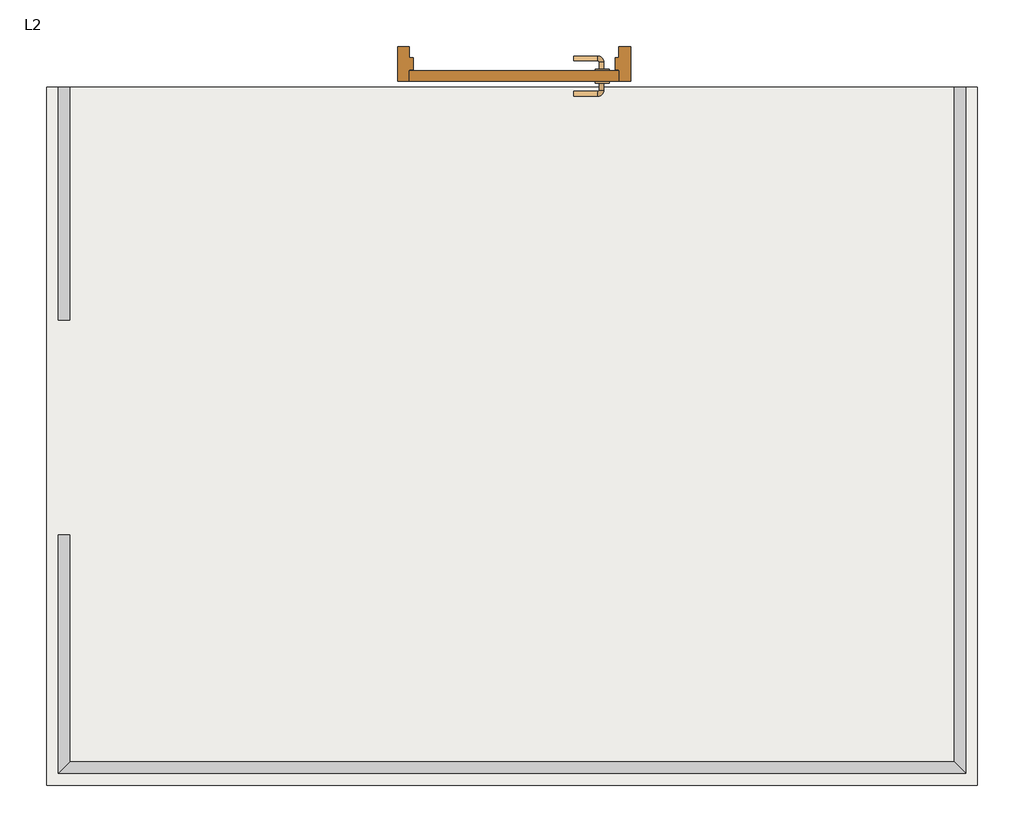
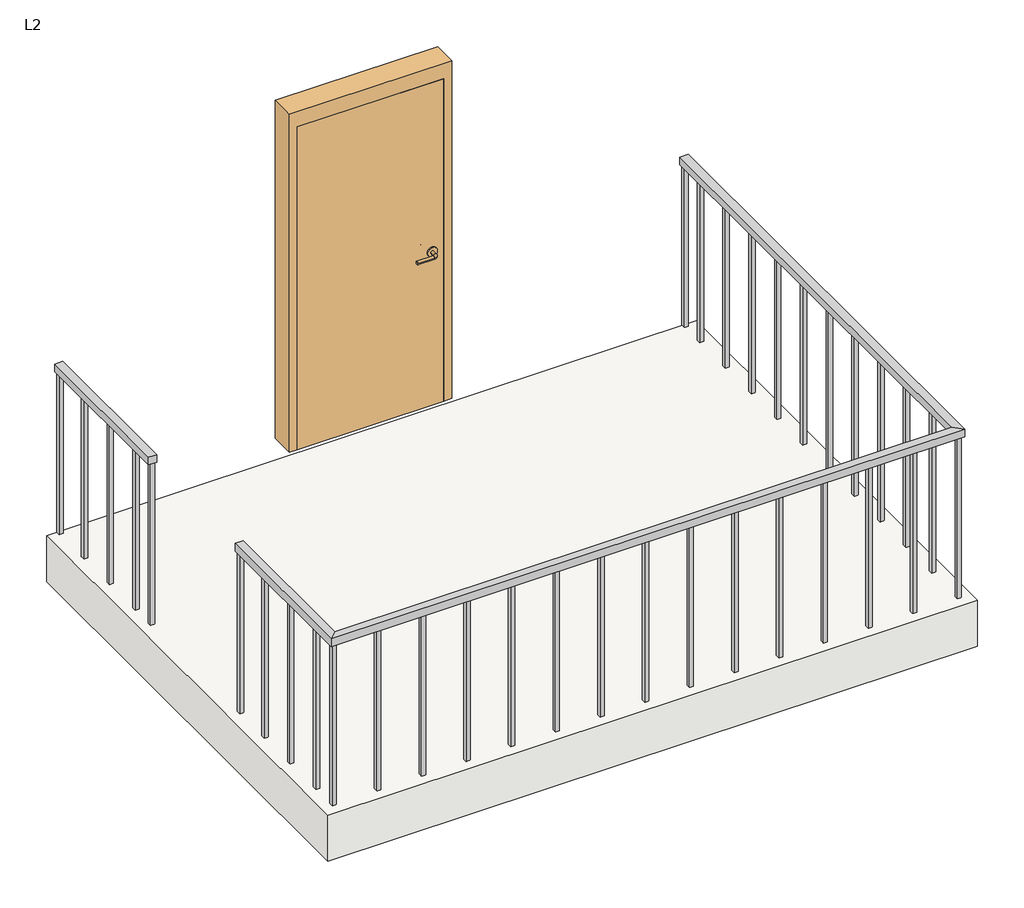
# One storey: 2 railings, 1 door, 1 slab.
"""IFC4 building model written with IfcOpenShell, lengths in millimetres."""

import ifcopenshell
import ifcopenshell.guid

model = None  # the IFC model being written
_history = None  # IfcOwnerHistory: only IFC2X3 demands one
_inside = {}  # id of a spatial element -> (the spatial element, [elements in it])
_under = {}  # id of a project, library or spatial element -> (it, [spatial elements below it])
_declared = {}  # id of a project -> (the project, [libraries it declares])
_typed = {}  # id of a type object -> (the type object, [elements of that type])
_made_of = {}  # id of a material, layer set ... -> (it, [elements and type objects made of it])


def new_model(schema):
    """Start an empty IFC model of exactly this schema.

    Asked for "IFC4X3", IfcOpenShell would pick the latest addendum, in which some entities
    have other attributes; the version numbers below select the first issue.
    IFC2X3 requires an IfcOwnerHistory on every rooted entity: one is made here for all.
    """
    global model, _history
    if schema == "IFC4X3":
        model = ifcopenshell.file(schema_version=(4, 3, 0, 0))
    else:
        model = ifcopenshell.file(schema=schema)
    _inside.clear()
    _under.clear()
    _declared.clear()
    _typed.clear()
    _made_of.clear()
    _history = None
    if model.schema == "IFC2X3":
        org = make("IfcOrganization", Name="unknown")
        user = make(
            "IfcPersonAndOrganization",
            ThePerson=make("IfcPerson", FamilyName="unknown"),
            TheOrganization=org,
        )
        app = make(
            "IfcApplication",
            ApplicationDeveloper=org,
            Version="unknown",
            ApplicationFullName="unknown",
            ApplicationIdentifier="unknown",
        )
        _history = make(
            "IfcOwnerHistory",
            OwningUser=user,
            OwningApplication=app,
            ChangeAction="ADDED",
            CreationDate=0,
        )
    return model


def make(cls, **values):
    """One entity of the class cls with the attributes given. An attribute that is None is left unset."""
    return model.create_entity(
        cls, **{name: value for name, value in values.items() if value is not None}
    )


def rooted(cls, **values):
    """An entity with a GlobalId (a new one), such as an element, a storey or a relation."""
    return make(cls, GlobalId=ifcopenshell.guid.new(), OwnerHistory=_history, **values)


def si_unit(unit_type, name, prefix=None):
    """IfcSIUnit, for example si_unit("LENGTHUNIT", "METRE", prefix="MILLI")."""
    return make("IfcSIUnit", UnitType=unit_type, Prefix=prefix, Name=name)


def assignment(units):
    """IfcUnitAssignment: the units of a project."""
    return None if units is None else make("IfcUnitAssignment", Units=units)


def point(xyz):
    """IfcCartesianPoint."""
    return None if xyz is None else make("IfcCartesianPoint", Coordinates=xyz)


def direction(xyz):
    """IfcDirection."""
    return None if xyz is None else make("IfcDirection", DirectionRatios=xyz)


def frame(location, z_axis=None, x_axis=None):
    """IfcAxis2Placement3D, a coordinate frame: its origin and axes. An axis left out is left unset."""
    return make(
        "IfcAxis2Placement3D",
        Location=point(location),
        Axis=direction(z_axis),
        RefDirection=direction(x_axis),
    )


def frame_2d(location, x_axis=None):
    """IfcAxis2Placement2D, a coordinate frame in the plane: its origin and x axis."""
    return make(
        "IfcAxis2Placement2D", Location=point(location), RefDirection=direction(x_axis)
    )


def origin():
    """The frame at (0, 0, 0) with its axes left unset."""
    return frame((0.0, 0.0, 0.0))


def origin_with_axes():
    """The frame at (0, 0, 0) with the z axis (0, 0, 1) and the x axis (1, 0, 0) written out."""
    return frame((0.0, 0.0, 0.0), z_axis=(0.0, 0.0, 1.0), x_axis=(1.0, 0.0, 0.0))


def place(relative_to, where):
    """IfcLocalPlacement: puts the frame where relative to a parent placement (None: the world)."""
    return make(
        "IfcLocalPlacement", PlacementRelTo=relative_to, RelativePlacement=where
    )


def context(
    kind, dimensions, precision=None, world=None, true_north=None, identifier=None
):
    """IfcGeometricRepresentationContext, for example the 3D "Model" context."""
    return make(
        "IfcGeometricRepresentationContext",
        ContextIdentifier=identifier,
        ContextType=kind,
        CoordinateSpaceDimension=dimensions,
        Precision=precision,
        WorldCoordinateSystem=world,
        TrueNorth=true_north,
    )


def project(units=None, contexts=None):
    """IfcProject with its units and contexts."""
    return rooted(
        "IfcProject",
        Name="project",
        RepresentationContexts=contexts,
        UnitsInContext=assignment(units),
    )


def spatial(cls, under=None, at=None, **own):
    """A site, building, storey or space (cls), placed at a placement, below another one or the project."""
    s = rooted(cls, ObjectPlacement=at, **own)
    if under is not None:
        _under.setdefault(under.id(), (under, []))[1].append(s)
    return s


def polyline(points):
    """IfcPolyline through the points."""
    return make("IfcPolyline", Points=[point(p) for p in points])


def circle_curve(where, radius):
    """IfcCircle in the frame where."""
    return make("IfcCircle", Position=where, Radius=radius)


def ellipse_curve(where, semi_axis1, semi_axis2):
    """IfcEllipse in the frame where."""
    return make(
        "IfcEllipse", Position=where, SemiAxis1=semi_axis1, SemiAxis2=semi_axis2
    )


def trimmed(basis, trim1, trim2, sense, master):
    """IfcTrimmedCurve: the piece of a basis curve between two trims."""
    return make(
        "IfcTrimmedCurve",
        BasisCurve=basis,
        Trim1=trim1,
        Trim2=trim2,
        SenseAgreement=sense,
        MasterRepresentation=master,
    )


def segment(curve, same_sense, transition):
    """IfcCompositeCurveSegment."""
    return make(
        "IfcCompositeCurveSegment",
        Transition=transition,
        SameSense=same_sense,
        ParentCurve=curve,
    )


def composite_curve(segments, self_intersect=None):
    """IfcCompositeCurve: segments joined end to end."""
    return make("IfcCompositeCurve", Segments=segments, SelfIntersect=self_intersect)


def outline(outer, holes=None, kind="AREA"):
    """IfcArbitraryClosedProfileDef: a profile drawn as a closed curve; with holes, ...WithVoids."""
    if holes is None:
        return make("IfcArbitraryClosedProfileDef", ProfileType=kind, OuterCurve=outer)
    return make(
        "IfcArbitraryProfileDefWithVoids",
        ProfileType=kind,
        OuterCurve=outer,
        InnerCurves=holes,
    )


def extrude(swept, where, along, depth):
    """IfcExtrudedAreaSolid: the profile swept, set in the frame where, extruded along a direction by depth."""
    return make(
        "IfcExtrudedAreaSolid",
        SweptArea=swept,
        Position=where,
        ExtrudedDirection=direction(along),
        Depth=depth,
    )


def faces_of(points, faces, orient=None, outer=None):
    """IfcFace entities. A face is a list of loops; a loop is a list of indices into points, from 0.

    orient and outer hold one flag for each loop. By default every Orientation is true, the
    first loop of a face is its IfcFaceOuterBound and the others are IfcFaceBound.
    """
    made = []
    for i, loops in enumerate(faces):
        bounds = []
        for j, loop in enumerate(loops):
            is_outer = j == 0 if outer is None else outer[i][j]
            bounds.append(
                make(
                    "IfcFaceOuterBound" if is_outer else "IfcFaceBound",
                    Bound=make("IfcPolyLoop", Polygon=[points[k] for k in loop]),
                    Orientation=True if orient is None else orient[i][j],
                )
            )
        made.append(make("IfcFace", Bounds=bounds))
    return made


def faceted_brep(points, faces, orient=None, outer=None, voids=None):
    """IfcFacetedBrep: a solid bounded by flat faces; with voids (closed shells), ...WithVoids."""
    shared = [point(p) for p in points]
    hull = make("IfcClosedShell", CfsFaces=faces_of(shared, faces, orient, outer))
    if voids is None:
        return make("IfcFacetedBrep", Outer=hull)
    return make(
        "IfcFacetedBrepWithVoids",
        Outer=hull,
        Voids=[
            make(cls, CfsFaces=faces_of(shared, fs, o, b)) for cls, fs, o, b in voids
        ],
    )


def shape(context_of_items, identifier, shape_type, items):
    """IfcShapeRepresentation: the items that make up one representation, for example the "Body"."""
    return make(
        "IfcShapeRepresentation",
        ContextOfItems=context_of_items,
        RepresentationIdentifier=identifier,
        RepresentationType=shape_type,
        Items=items,
    )


def source(mapping_origin, context_of_items, identifier, shape_type, items):
    """IfcRepresentationMap: a shape defined once, which mapped items show again and again."""
    return make(
        "IfcRepresentationMap",
        MappingOrigin=mapping_origin,
        MappedRepresentation=shape(context_of_items, identifier, shape_type, items),
    )


def transform(
    local_origin,
    x_axis=None,
    y_axis=None,
    z_axis=None,
    scale=None,
    scale2=None,
    scale3=None,
    uniform=True,
):
    """IfcCartesianTransformationOperator3D, or its non-uniform kind. x_axis, y_axis, z_axis: its Axis1, 2, 3."""
    if uniform:
        return make(
            "IfcCartesianTransformationOperator3D",
            Axis1=direction(x_axis),
            Axis2=direction(y_axis),
            LocalOrigin=point(local_origin),
            Scale=scale,
            Axis3=direction(z_axis),
        )
    return make(
        "IfcCartesianTransformationOperator3DnonUniform",
        Axis1=direction(x_axis),
        Axis2=direction(y_axis),
        LocalOrigin=point(local_origin),
        Scale=scale,
        Axis3=direction(z_axis),
        Scale2=scale2,
        Scale3=scale3,
    )


def mapped(mapping_source, mapping_target):
    """IfcMappedItem: shows the shape of a source again, moved by a transform."""
    return make(
        "IfcMappedItem", MappingSource=mapping_source, MappingTarget=mapping_target
    )


def made_of(thing, what):
    """Note that an element or type object is made of a material, layer set ...; save() writes the relation."""
    if what is not None:
        _made_of.setdefault(what.id(), (what, []))[1].append(thing)
    return thing


def element(
    cls,
    number,
    at=None,
    inside=None,
    cuts=None,
    type_object=None,
    material=None,
    context=None,
    identifier="Body",
    shape_type=None,
    held_by="IfcProductDefinitionShape",
    body=None,
    shapes=None,
    **own,
):
    """One element of the class cls, such as IfcWall. Its Tag is "e" and its number.

    at: its placement. inside: the storey or other place that contains it. cuts: it is an
    opening in that element (IfcRelVoidsElement). A single representation is given by context,
    identifier, shape_type and body (its items); several are given by shapes. held_by: the class
    of the entity that holds the representations. save() writes the other relations.
    """
    e = rooted(cls, Tag="e%d" % number, ObjectPlacement=at, **own)
    if body is not None:
        shapes = [shape(context, identifier, shape_type, body)]
    if shapes is not None:
        e.Representation = make(held_by, Representations=shapes)
    if inside is not None:
        _inside.setdefault(inside.id(), (inside, []))[1].append(e)
    if cuts is not None:
        rooted(
            "IfcRelVoidsElement", RelatingBuildingElement=cuts, RelatedOpeningElement=e
        )
    if type_object is not None:
        _typed.setdefault(type_object.id(), (type_object, []))[1].append(e)
    return made_of(e, material)


def aggregate(whole, parts):
    """IfcRelAggregates: a whole, such as a stair, and the parts it consists of."""
    return rooted("IfcRelAggregates", RelatingObject=whole, RelatedObjects=parts)


def save(model, path):
    """Write the relations noted so far, then the file.

    IfcRelAggregates (storeys below a building ...), IfcRelContainedInSpatialStructure (elements
    in a storey), IfcRelDefinesByType, IfcRelAssociatesMaterial and IfcRelDeclares: one each for
    every whole, place, type object, material and project.
    """
    for whole, parts in _under.values():
        aggregate(whole, parts)
    for where, things in _inside.values():
        rooted(
            "IfcRelContainedInSpatialStructure",
            RelatedElements=things,
            RelatingStructure=where,
        )
    for kind, things in _typed.values():
        rooted("IfcRelDefinesByType", RelatedObjects=things, RelatingType=kind)
    for what, things in _made_of.values():
        rooted("IfcRelAssociatesMaterial", RelatedObjects=things, RelatingMaterial=what)
    for by, libraries in _declared.values():
        rooted("IfcRelDeclares", RelatingContext=by, RelatedDefinitions=libraries)
    model.write(path)


def plane_surface(at):
    """IfcPlane: the flat surface through the origin of the frame at, square to its z axis."""
    return make("IfcPlane", Position=at)


def cylinder_surface(at, radius):
    """IfcCylindricalSurface: all points at the distance radius from the z axis of the frame at."""
    return make("IfcCylindricalSurface", Position=at, Radius=radius)


def revolved_surface(curve, axis_point, axis_direction):
    """IfcSurfaceOfRevolution: the curve turned about the line through axis_point along axis_direction."""
    return make(
        "IfcSurfaceOfRevolution",
        SweptCurve=make("IfcArbitraryOpenProfileDef", ProfileType="CURVE", Curve=curve),
        AxisPosition=make("IfcAxis1Placement", Location=point(axis_point), Axis=direction(axis_direction)),
    )


def advanced_brep(points, edges, surfaces, faces):
    """IfcAdvancedBrep: a solid bounded by faces that lie on surfaces and meet in shared edges.

    An edge is (start, end): straight between two places in points (the first is 0);
    or (start, end, curve); or (start, end, curve, False) where it runs against its curve.
    A face is (place in surfaces, loops), or (place, loops, False) where it looks against
    its surface's normal. A loop lists edges by number (the first is 1), with a minus sign
    where the edge is run from its end to its start. The first loop is the outer one.
    """
    corners = [point(p) for p in points]
    vertices = [make("IfcVertexPoint", VertexGeometry=c) for c in corners]
    made = []
    for start, end, *more in edges:
        made.append(
            make(
                "IfcEdgeCurve",
                EdgeStart=vertices[start],
                EdgeEnd=vertices[end],
                EdgeGeometry=more[0] if more else make("IfcPolyline", Points=[corners[start], corners[end]]),
                SameSense=more[1] if len(more) > 1 else True,
            )
        )
    hull = []
    for where, loops, *sense in faces:
        bounds = []
        for j, loop in enumerate(loops):
            ring = [make("IfcOrientedEdge", EdgeElement=made[abs(k) - 1], Orientation=k > 0) for k in loop]
            bounds.append(
                make(
                    "IfcFaceOuterBound" if j == 0 else "IfcFaceBound",
                    Bound=make("IfcEdgeLoop", EdgeList=ring),
                    Orientation=True,
                )
            )
        hull.append(make("IfcAdvancedFace", Bounds=bounds, FaceSurface=surfaces[where], SameSense=sense[0] if sense else True))
    return make("IfcAdvancedBrep", Outer=make("IfcClosedShell", CfsFaces=hull))


def m_door_passage_single_flush_900_x_2100mm_f70d95c9(model_context):
    return source(origin(), model_context, "Body", "SolidModel", [
        advanced_brep(
        [(-384.990625, 3.35, 1000.0), (-364.990625, 3.35, 1000.0), (-364.990625, -26.65, 1000.0), (-384.990625, -26.65, 1000.0), (-359.990625, -31.65, 1000.0), (-359.990625, -51.65, 1000.0), (-254.990625, -51.65, 1000.0), (-254.990625, -31.65, 1000.0)],
        [
            (0, 1, circle_curve(frame((-374.990625, 3.35, 1000.0), z_axis=(0.0, 1.0, 0.0), x_axis=(1.0, 0.0, 0.0)), 10.0)),
            (1, 0, circle_curve(frame((-374.990625, 3.35, 1000.0), z_axis=(0.0, 1.0, 0.0), x_axis=(1.0, 0.0, 0.0)), 10.0)),
            (1, 2),
            (2, 3, circle_curve(frame((-374.990625, -26.65, 1000.0), z_axis=(0.0, 1.0, 0.0), x_axis=(1.0, 0.0, 0.0)), 10.0)),
            (3, 0),
            (3, 2, circle_curve(frame((-374.990625, -26.65, 1000.0), z_axis=(0.0, 1.0, 0.0), x_axis=(1.0, 0.0, 0.0)), 10.0)),
            (4, 5, circle_curve(frame((-359.990625, -41.65, 1000.0), z_axis=(-1.0, 0.0, 0.0), x_axis=(0.0, 1.0, 0.0)), 10.0)),
            (5, 3, circle_curve(frame((-359.990625, -26.65, 1000.0), z_axis=(0.0, 0.0, -1.0), x_axis=(-1.0, 0.0, 0.0)), 25.0)),
            (2, 4, circle_curve(frame((-359.990625, -26.65, 1000.0), z_axis=(0.0, 0.0, 1.0), x_axis=(-1.0, 0.0, 0.0)), 5.0)),
            (5, 4, circle_curve(frame((-359.990625, -41.65, 1000.0), z_axis=(-1.0, 0.0, 0.0), x_axis=(0.0, 1.0, 0.0)), 10.0)),
            (6, 7, circle_curve(frame((-254.990625, -41.65, 1000.0), z_axis=(1.0, 0.0, 0.0), x_axis=(0.0, 1.0, 0.0)), 10.0)),
            (7, 6, circle_curve(frame((-254.990625, -41.65, 1000.0), z_axis=(1.0, 0.0, 0.0), x_axis=(0.0, 1.0, 0.0)), 10.0)),
            (4, 7),
            (6, 5),
        ],
        [
            plane_surface(frame((-374.990625, 3.35, 1000.0), z_axis=(0.0, 1.0, 0.0), x_axis=(0.0, 0.0, 1.0))),
            cylinder_surface(frame((-374.990625, 3.35, 1000.0), z_axis=(0.0, 1.0, 0.0), x_axis=(1.0, 0.0, 0.0)), 10.0),
            revolved_surface(trimmed(ellipse_curve(frame((-374.990625, -26.65, 1000.0), z_axis=(0.0, -1.0, 0.0), x_axis=(1.0, 0.0, 0.0)), 10.0, 10.0), [point((-384.990625, -26.65, 1000.0))], [point((-364.990625, -26.65, 1000.0))], True, "CARTESIAN"), (-359.990625, -26.65, 1000.0), (0.0, 0.0, -1.0)),
            revolved_surface(trimmed(ellipse_curve(frame((-374.990625, -26.65, 1000.0), z_axis=(0.0, -1.0, 0.0), x_axis=(1.0, 0.0, 0.0)), 10.0, 10.0), [point((-364.990625, -26.65, 1000.0))], [point((-384.990625, -26.65, 1000.0))], True, "CARTESIAN"), (-359.990625, -26.65, 1000.0), (0.0, 0.0, -1.0)),
            plane_surface(frame((-254.990625, -41.65, 1000.0), z_axis=(1.0, 0.0, 0.0), x_axis=(0.0, 0.0, 1.0))),
            cylinder_surface(frame((-359.990625, -41.65, 1000.0), z_axis=(-1.0, 0.0, 0.0), x_axis=(0.0, 1.0, 0.0)), 10.0),
        ],
        [
            (0, [[1, 2]]),
            (1, [[3, 4, 5, -2]]),
            (1, [[-5, 6, -3, -1]]),
            (2, [[7, 8, -4, 9]]),
            (3, [[10, -9, -6, -8]]),
            (4, [[11, 12]]),
            (5, [[13, -11, 14, -7]]),
            (5, [[-14, -12, -13, -10]]),
        ],
    ),
        extrude(outline(composite_curve([segment(trimmed(circle_curve(frame_2d((1000.0, -377.490625)), 30.0), [point((1000.0, -407.490625))], [point((1000.0, -347.490625))], False, "CARTESIAN"), True, "CONTINUOUS"), segment(trimmed(circle_curve(frame_2d((1000.0, -377.490625)), 30.0), [point((1000.0, -347.490625))], [point((1000.0, -407.490625))], False, "CARTESIAN"), True, "CONTINUOUS")], self_intersect=False)), frame((0.0, 3.35, 0.0), z_axis=(0.0, 1.0, 0.0), x_axis=(0.0, 0.0, 1.0)), (0.0, 0.0, 1.0), 8.0),
        advanced_brep(
        [(-384.990625, 64.35, 1000.0), (-364.990625, 64.35, 1000.0), (-384.990625, 94.35, 1000.0), (-364.990625, 94.35, 1000.0), (-359.990625, 99.35, 1000.0), (-359.990625, 119.35, 1000.0), (-254.990625, 119.35, 1000.0), (-254.990625, 99.35, 1000.0)],
        [
            (0, 1, circle_curve(frame((-374.990625, 64.35, 1000.0), z_axis=(0.0, -1.0, 0.0), x_axis=(1.0, 0.0, 0.0)), 10.0)),
            (1, 0, circle_curve(frame((-374.990625, 64.35, 1000.0), z_axis=(0.0, -1.0, 0.0), x_axis=(1.0, 0.0, 0.0)), 10.0)),
            (0, 2),
            (2, 3, circle_curve(frame((-374.990625, 94.35, 1000.0), z_axis=(0.0, -1.0, 0.0), x_axis=(1.0, 0.0, 0.0)), 10.0)),
            (3, 1),
            (3, 2, circle_curve(frame((-374.990625, 94.35, 1000.0), z_axis=(0.0, -1.0, 0.0), x_axis=(1.0, 0.0, 0.0)), 10.0)),
            (4, 3, circle_curve(frame((-359.990625, 94.35, 1000.0), z_axis=(0.0, 0.0, 1.0), x_axis=(-1.0, 0.0, 0.0)), 5.0)),
            (2, 5, circle_curve(frame((-359.990625, 94.35, 1000.0), z_axis=(0.0, 0.0, -1.0), x_axis=(-1.0, 0.0, 0.0)), 25.0)),
            (5, 4, circle_curve(frame((-359.990625, 109.35, 1000.0), z_axis=(-1.0, 0.0, 0.0), x_axis=(0.0, -1.0, 0.0)), 10.0)),
            (4, 5, circle_curve(frame((-359.990625, 109.35, 1000.0), z_axis=(-1.0, 0.0, 0.0), x_axis=(0.0, -1.0, 0.0)), 10.0)),
            (6, 7, circle_curve(frame((-254.990625, 109.35, 1000.0), z_axis=(1.0, 0.0, 0.0), x_axis=(0.0, -1.0, 0.0)), 10.0)),
            (7, 6, circle_curve(frame((-254.990625, 109.35, 1000.0), z_axis=(1.0, 0.0, 0.0), x_axis=(0.0, -1.0, 0.0)), 10.0)),
            (5, 6),
            (7, 4),
        ],
        [
            plane_surface(frame((-374.990625, 64.35, 1000.0), z_axis=(0.0, -1.0, 0.0), x_axis=(0.0, 0.0, 1.0))),
            cylinder_surface(frame((-374.990625, 64.35, 1000.0), z_axis=(0.0, -1.0, 0.0), x_axis=(1.0, 0.0, 0.0)), 10.0),
            revolved_surface(trimmed(ellipse_curve(frame((-374.990625, 94.35, 1000.0), z_axis=(0.0, -1.0, 0.0), x_axis=(1.0, 0.0, 0.0)), 10.0, 10.0), [point((-384.990625, 94.35, 1000.0))], [point((-364.990625, 94.35, 1000.0))], True, "CARTESIAN"), (-359.990625, 94.35, 1000.0), (0.0, 0.0, -1.0)),
            revolved_surface(trimmed(ellipse_curve(frame((-374.990625, 94.35, 1000.0), z_axis=(0.0, -1.0, 0.0), x_axis=(1.0, 0.0, 0.0)), 10.0, 10.0), [point((-364.990625, 94.35, 1000.0))], [point((-384.990625, 94.35, 1000.0))], True, "CARTESIAN"), (-359.990625, 94.35, 1000.0), (0.0, 0.0, -1.0)),
            plane_surface(frame((-254.990625, 109.35, 1000.0), z_axis=(1.0, 0.0, 0.0), x_axis=(0.0, 0.0, 1.0))),
            cylinder_surface(frame((-359.990625, 109.35, 1000.0), z_axis=(-1.0, 0.0, 0.0), x_axis=(0.0, -1.0, 0.0)), 10.0),
        ],
        [
            (0, [[1, 2]]),
            (1, [[-1, 3, 4, 5]]),
            (1, [[-2, -5, 6, -3]]),
            (2, [[7, -4, 8, 9]]),
            (3, [[-8, -6, -7, 10]]),
            (4, [[11, 12]]),
            (5, [[-9, 13, -12, 14]]),
            (5, [[-10, -14, -11, -13]]),
        ],
    ),
        extrude(outline(composite_curve([segment(trimmed(circle_curve(frame_2d((1000.0, -377.490625)), 30.0), [point((1000.0, -407.490625))], [point((1000.0, -347.490625))], False, "CARTESIAN"), True, "CONTINUOUS"), segment(trimmed(circle_curve(frame_2d((1000.0, -377.490625)), 30.0), [point((1000.0, -347.490625))], [point((1000.0, -407.490625))], False, "CARTESIAN"), True, "CONTINUOUS")], self_intersect=False)), frame((0.0, 56.35, 0.0), z_axis=(0.0, 1.0, 0.0), x_axis=(0.0, 0.0, 1.0)), (0.0, 0.0, 1.0), 8.0),
        extrude(outline(polyline([(450.0, 11.35), (-450.0, 11.35), (-450.0, 56.35), (450.0, 56.35), (450.0, 11.35)])), origin_with_axes(), (0.0, 0.0, 1.0), 2100.0),
        faceted_brep([(450.0, 6.5875, 0.0), (450.0, 56.35, 0.0), (500.0, 56.35, 0.0), (500.0, -93.65, 0.0), (450.0, -93.65, 0.0), (450.0, -44.4375, 0.0), (434.125, -44.4375, 0.0), (434.125, 6.5875, 0.0), (450.0, 6.5875, 2100.0), (450.0, 56.35, 2100.0), (-450.0, 56.35, 2100.0), (-450.0, 56.35, 0.0), (-500.0, 56.35, 0.0), (-500.0, 56.35, 2200.0), (500.0, 56.35, 2200.0), (500.0, -93.65, 2200.0), (-500.0, -93.65, 2200.0), (-500.0, -93.65, 0.0), (-450.0, -93.65, 0.0), (-450.0, -93.65, 2100.0), (450.0, -93.65, 2100.0), (450.0, -44.4375, 2100.0), (-450.0, -44.4375, 2100.0), (-450.0, -44.4375, 0.0), (-434.125, -44.4375, 0.0), (-434.125, -44.4375, 2084.125), (434.125, -44.4375, 2084.125), (434.125, 6.5875, 2084.125), (-434.125, 6.5875, 2084.125), (-434.125, 6.5875, 0.0), (-450.0, 6.5875, 0.0), (-450.0, 6.5875, 2100.0)], [[[0, 1, 2, 3, 4, 5, 6, 7]], [[1, 0, 8, 9]], [[2, 1, 9, 10, 11, 12, 13, 14]], [[3, 2, 14, 15]], [[4, 3, 15, 16, 17, 18, 19, 20]], [[5, 4, 20, 21]], [[6, 5, 21, 22, 23, 24, 25, 26]], [[7, 6, 26, 27]], [[0, 7, 27, 28, 29, 30, 31, 8]], [[9, 8, 31, 10]], [[20, 19, 22, 21]], [[26, 25, 28, 27]], [[12, 11, 30, 29, 24, 23, 18, 17]], [[11, 10, 31, 30]], [[13, 12, 17, 16]], [[19, 18, 23, 22]], [[25, 24, 29, 28]], [[15, 14, 13, 16]]]),
    ])


model = new_model("IFC4")

# Units and contexts
model_context = context("Model", 3, world=origin())
ifc_project = project(units=[si_unit("LENGTHUNIT", "METRE", prefix="MILLI")], contexts=[model_context])

# Site, building, storey
site = spatial("IfcSite", under=ifc_project)
building = spatial("IfcBuilding", under=site)
storey = spatial("IfcBuildingStorey", under=building, Name="L2", Elevation=1200.0)

# Door
placement = place(None, origin())
m_door_passage_single_flush_900_x_2100mm_shape = m_door_passage_single_flush_900_x_2100mm_f70d95c9(model_context)
element("IfcDoor", 1, ObjectType="M_Door-Passage-Single-Flush : 900 x 2100mm", at=placement, inside=storey, context=model_context, shape_type="MappedRepresentation", body=[
    mapped(m_door_passage_single_flush_900_x_2100mm_shape, transform((752.7568, 2222.9207088, 1200.0), x_axis=(-1.0, 0.0, 0.0), y_axis=(0.0, -1.0, 0.0), z_axis=(0.0, 0.0, 1.0))),
])

# Railings
element("IfcRailing", 2, ObjectType="1100mm", at=placement, inside=storey, context=model_context, shape_type="SolidModel", body=[
    faceted_brep([(-1156.7682, 216.5707088, 2300.0), (-1156.7682, 216.5707088, 2250.0), (-1206.7682, 216.5707088, 2250.0), (-1206.7682, 216.5707088, 2300.0), (-1156.7682, -758.4292912, 2300.0), (-1156.7682, -758.4292912, 2250.0), (-1206.7682, -808.4292912, 2250.0), (-1206.7682, -808.4292912, 2300.0), (2643.2318, -758.4292912, 2300.0), (2643.2318, -758.4292912, 2250.0), (2693.2318, -808.4292912, 2250.0), (2693.2318, -808.4292912, 2300.0), (2643.2318, 2141.5707088, 2300.0), (2693.2318, 2141.5707088, 2300.0), (2693.2318, 2141.5707088, 2250.0), (2643.2318, 2141.5707088, 2250.0)], [[[0, 1, 2, 3]], [[1, 0, 4, 5]], [[2, 1, 5, 6]], [[3, 2, 6, 7]], [[0, 3, 7, 4]], [[5, 4, 8, 9]], [[6, 5, 9, 10]], [[7, 6, 10, 11]], [[4, 7, 11, 8]], [[12, 13, 14, 15]], [[9, 8, 12, 15]], [[10, 9, 15, 14]], [[11, 10, 14, 13]], [[8, 11, 13, 12]]]),
    extrude(outline(polyline([(2680.7318, 1954.0707088), (2655.7318, 1954.0707088), (2655.7318, 1979.0707088), (2680.7318, 1979.0707088), (2680.7318, 1954.0707088)])), frame((0.0, 0.0, 1200.0), z_axis=(0.0, 0.0, 1.0), x_axis=(1.0, 0.0, 0.0)), (0.0, 0.0, 1.0), 1050.0),
    extrude(outline(polyline([(2680.7318, 1679.0707088), (2655.7318, 1679.0707088), (2655.7318, 1704.0707088), (2680.7318, 1704.0707088), (2680.7318, 1679.0707088)])), frame((0.0, 0.0, 1200.0), z_axis=(0.0, 0.0, 1.0), x_axis=(1.0, 0.0, 0.0)), (0.0, 0.0, 1.0), 1050.0),
    extrude(outline(polyline([(2680.7318, 1404.0707088), (2655.7318, 1404.0707088), (2655.7318, 1429.0707088), (2680.7318, 1429.0707088), (2680.7318, 1404.0707088)])), frame((0.0, 0.0, 1200.0), z_axis=(0.0, 0.0, 1.0), x_axis=(1.0, 0.0, 0.0)), (0.0, 0.0, 1.0), 1050.0),
    extrude(outline(polyline([(2680.7318, 1129.0707088), (2655.7318, 1129.0707088), (2655.7318, 1154.0707088), (2680.7318, 1154.0707088), (2680.7318, 1129.0707088)])), frame((0.0, 0.0, 1200.0), z_axis=(0.0, 0.0, 1.0), x_axis=(1.0, 0.0, 0.0)), (0.0, 0.0, 1.0), 1050.0),
    extrude(outline(polyline([(2680.7318, 854.0707088), (2655.7318, 854.0707088), (2655.7318, 879.0707088), (2680.7318, 879.0707088), (2680.7318, 854.0707088)])), frame((0.0, 0.0, 1200.0), z_axis=(0.0, 0.0, 1.0), x_axis=(1.0, 0.0, 0.0)), (0.0, 0.0, 1.0), 1050.0),
    extrude(outline(polyline([(2680.7318, 579.0707088), (2655.7318, 579.0707088), (2655.7318, 604.0707088), (2680.7318, 604.0707088), (2680.7318, 579.0707088)])), frame((0.0, 0.0, 1200.0), z_axis=(0.0, 0.0, 1.0), x_axis=(1.0, 0.0, 0.0)), (0.0, 0.0, 1.0), 1050.0),
    extrude(outline(polyline([(2680.7318, 304.0707088), (2655.7318, 304.0707088), (2655.7318, 329.0707088), (2680.7318, 329.0707088), (2680.7318, 304.0707088)])), frame((0.0, 0.0, 1200.0), z_axis=(0.0, 0.0, 1.0), x_axis=(1.0, 0.0, 0.0)), (0.0, 0.0, 1.0), 1050.0),
    extrude(outline(polyline([(2680.7318, 29.0707088), (2655.7318, 29.0707088), (2655.7318, 54.0707088), (2680.7318, 54.0707088), (2680.7318, 29.0707088)])), frame((0.0, 0.0, 1200.0), z_axis=(0.0, 0.0, 1.0), x_axis=(1.0, 0.0, 0.0)), (0.0, 0.0, 1.0), 1050.0),
    extrude(outline(polyline([(2680.7318, -245.9292912), (2655.7318, -245.9292912), (2655.7318, -220.9292912), (2680.7318, -220.9292912), (2680.7318, -245.9292912)])), frame((0.0, 0.0, 1200.0), z_axis=(0.0, 0.0, 1.0), x_axis=(1.0, 0.0, 0.0)), (0.0, 0.0, 1.0), 1050.0),
    extrude(outline(polyline([(2680.7318, -520.9292912), (2655.7318, -520.9292912), (2655.7318, -495.9292912), (2680.7318, -495.9292912), (2680.7318, -520.9292912)])), frame((0.0, 0.0, 1200.0), z_axis=(0.0, 0.0, 1.0), x_axis=(1.0, 0.0, 0.0)), (0.0, 0.0, 1.0), 1050.0),
    extrude(outline(polyline([(2380.7318, -795.9292912), (2380.7318, -770.9292912), (2405.7318, -770.9292912), (2405.7318, -795.9292912), (2380.7318, -795.9292912)])), frame((0.0, 0.0, 1200.0), z_axis=(0.0, 0.0, 1.0), x_axis=(1.0, 0.0, 0.0)), (0.0, 0.0, 1.0), 1050.0),
    extrude(outline(polyline([(2105.7318, -795.9292912), (2105.7318, -770.9292912), (2130.7318, -770.9292912), (2130.7318, -795.9292912), (2105.7318, -795.9292912)])), frame((0.0, 0.0, 1200.0), z_axis=(0.0, 0.0, 1.0), x_axis=(1.0, 0.0, 0.0)), (0.0, 0.0, 1.0), 1050.0),
    extrude(outline(polyline([(1830.7318, -795.9292912), (1830.7318, -770.9292912), (1855.7318, -770.9292912), (1855.7318, -795.9292912), (1830.7318, -795.9292912)])), frame((0.0, 0.0, 1200.0), z_axis=(0.0, 0.0, 1.0), x_axis=(1.0, 0.0, 0.0)), (0.0, 0.0, 1.0), 1050.0),
    extrude(outline(polyline([(1555.7318, -795.9292912), (1555.7318, -770.9292912), (1580.7318, -770.9292912), (1580.7318, -795.9292912), (1555.7318, -795.9292912)])), frame((0.0, 0.0, 1200.0), z_axis=(0.0, 0.0, 1.0), x_axis=(1.0, 0.0, 0.0)), (0.0, 0.0, 1.0), 1050.0),
    extrude(outline(polyline([(1280.7318, -795.9292912), (1280.7318, -770.9292912), (1305.7318, -770.9292912), (1305.7318, -795.9292912), (1280.7318, -795.9292912)])), frame((0.0, 0.0, 1200.0), z_axis=(0.0, 0.0, 1.0), x_axis=(1.0, 0.0, 0.0)), (0.0, 0.0, 1.0), 1050.0),
    extrude(outline(polyline([(1005.7318, -795.9292912), (1005.7318, -770.9292912), (1030.7318, -770.9292912), (1030.7318, -795.9292912), (1005.7318, -795.9292912)])), frame((0.0, 0.0, 1200.0), z_axis=(0.0, 0.0, 1.0), x_axis=(1.0, 0.0, 0.0)), (0.0, 0.0, 1.0), 1050.0),
    extrude(outline(polyline([(730.7318, -795.9292912), (730.7318, -770.9292912), (755.7318, -770.9292912), (755.7318, -795.9292912), (730.7318, -795.9292912)])), frame((0.0, 0.0, 1200.0), z_axis=(0.0, 0.0, 1.0), x_axis=(1.0, 0.0, 0.0)), (0.0, 0.0, 1.0), 1050.0),
    extrude(outline(polyline([(455.7318, -795.9292912), (455.7318, -770.9292912), (480.7318, -770.9292912), (480.7318, -795.9292912), (455.7318, -795.9292912)])), frame((0.0, 0.0, 1200.0), z_axis=(0.0, 0.0, 1.0), x_axis=(1.0, 0.0, 0.0)), (0.0, 0.0, 1.0), 1050.0),
    extrude(outline(polyline([(180.7318, -795.9292912), (180.7318, -770.9292912), (205.7318, -770.9292912), (205.7318, -795.9292912), (180.7318, -795.9292912)])), frame((0.0, 0.0, 1200.0), z_axis=(0.0, 0.0, 1.0), x_axis=(1.0, 0.0, 0.0)), (0.0, 0.0, 1.0), 1050.0),
    extrude(outline(polyline([(-94.2682, -795.9292912), (-94.2682, -770.9292912), (-69.2682, -770.9292912), (-69.2682, -795.9292912), (-94.2682, -795.9292912)])), frame((0.0, 0.0, 1200.0), z_axis=(0.0, 0.0, 1.0), x_axis=(1.0, 0.0, 0.0)), (0.0, 0.0, 1.0), 1050.0),
    extrude(outline(polyline([(-369.2682, -795.9292912), (-369.2682, -770.9292912), (-344.2682, -770.9292912), (-344.2682, -795.9292912), (-369.2682, -795.9292912)])), frame((0.0, 0.0, 1200.0), z_axis=(0.0, 0.0, 1.0), x_axis=(1.0, 0.0, 0.0)), (0.0, 0.0, 1.0), 1050.0),
    extrude(outline(polyline([(-644.2682, -795.9292912), (-644.2682, -770.9292912), (-619.2682, -770.9292912), (-619.2682, -795.9292912), (-644.2682, -795.9292912)])), frame((0.0, 0.0, 1200.0), z_axis=(0.0, 0.0, 1.0), x_axis=(1.0, 0.0, 0.0)), (0.0, 0.0, 1.0), 1050.0),
    extrude(outline(polyline([(-919.2682, -795.9292912), (-919.2682, -770.9292912), (-894.2682, -770.9292912), (-894.2682, -795.9292912), (-919.2682, -795.9292912)])), frame((0.0, 0.0, 1200.0), z_axis=(0.0, 0.0, 1.0), x_axis=(1.0, 0.0, 0.0)), (0.0, 0.0, 1.0), 1050.0),
    extrude(outline(polyline([(-1194.2682, -595.9292912), (-1169.2682, -595.9292912), (-1169.2682, -620.9292912), (-1194.2682, -620.9292912), (-1194.2682, -595.9292912)])), frame((0.0, 0.0, 1200.0), z_axis=(0.0, 0.0, 1.0), x_axis=(1.0, 0.0, 0.0)), (0.0, 0.0, 1.0), 1050.0),
    extrude(outline(polyline([(-1194.2682, -320.9292912), (-1169.2682, -320.9292912), (-1169.2682, -345.9292912), (-1194.2682, -345.9292912), (-1194.2682, -320.9292912)])), frame((0.0, 0.0, 1200.0), z_axis=(0.0, 0.0, 1.0), x_axis=(1.0, 0.0, 0.0)), (0.0, 0.0, 1.0), 1050.0),
    extrude(outline(polyline([(-1194.2682, -45.9292912), (-1169.2682, -45.9292912), (-1169.2682, -70.9292912), (-1194.2682, -70.9292912), (-1194.2682, -45.9292912)])), frame((0.0, 0.0, 1200.0), z_axis=(0.0, 0.0, 1.0), x_axis=(1.0, 0.0, 0.0)), (0.0, 0.0, 1.0), 1050.0),
    extrude(outline(polyline([(2655.7318, -795.9292912), (2655.7318, -770.9292912), (2680.7318, -770.9292912), (2680.7318, -795.9292912), (2655.7318, -795.9292912)])), frame((0.0, 0.0, 1200.0), z_axis=(0.0, 0.0, 1.0), x_axis=(1.0, 0.0, 0.0)), (0.0, 0.0, 1.0), 1050.0),
    extrude(outline(polyline([(-1194.2682, -770.9292912), (-1169.2682, -770.9292912), (-1169.2682, -795.9292912), (-1194.2682, -795.9292912), (-1194.2682, -770.9292912)])), frame((0.0, 0.0, 1200.0), z_axis=(0.0, 0.0, 1.0), x_axis=(1.0, 0.0, 0.0)), (0.0, 0.0, 1.0), 1050.0),
    extrude(outline(polyline([(2680.7318, 2116.5707088), (2655.7318, 2116.5707088), (2655.7318, 2141.5707088), (2680.7318, 2141.5707088), (2680.7318, 2116.5707088)])), frame((0.0, 0.0, 1200.0), z_axis=(0.0, 0.0, 1.0), x_axis=(1.0, 0.0, 0.0)), (0.0, 0.0, 1.0), 1050.0),
    extrude(outline(polyline([(-1194.2682, 216.5707088), (-1169.2682, 216.5707088), (-1169.2682, 191.5707088), (-1194.2682, 191.5707088), (-1194.2682, 216.5707088)])), frame((0.0, 0.0, 1200.0), z_axis=(0.0, 0.0, 1.0), x_axis=(1.0, 0.0, 0.0)), (0.0, 0.0, 1.0), 1050.0),
])
element("IfcRailing", 3, ObjectType="1100mm", at=placement, inside=storey, context=model_context, shape_type="SweptSolid", body=[
    extrude(outline(polyline([(-1206.7682, 2141.5707088), (-1156.7682, 2141.5707088), (-1156.7682, 1141.5707088), (-1206.7682, 1141.5707088), (-1206.7682, 2141.5707088)])), frame((0.0, 0.0, 2250.0), z_axis=(0.0, 0.0, 1.0), x_axis=(1.0, 0.0, 0.0)), (0.0, 0.0, 1.0), 50.0),
    extrude(outline(polyline([(-1194.2682, 1329.0707088), (-1169.2682, 1329.0707088), (-1169.2682, 1304.0707088), (-1194.2682, 1304.0707088), (-1194.2682, 1329.0707088)])), frame((0.0, 0.0, 1200.0), z_axis=(0.0, 0.0, 1.0), x_axis=(1.0, 0.0, 0.0)), (0.0, 0.0, 1.0), 1050.0),
    extrude(outline(polyline([(-1194.2682, 1604.0707088), (-1169.2682, 1604.0707088), (-1169.2682, 1579.0707088), (-1194.2682, 1579.0707088), (-1194.2682, 1604.0707088)])), frame((0.0, 0.0, 1200.0), z_axis=(0.0, 0.0, 1.0), x_axis=(1.0, 0.0, 0.0)), (0.0, 0.0, 1.0), 1050.0),
    extrude(outline(polyline([(-1194.2682, 1879.0707088), (-1169.2682, 1879.0707088), (-1169.2682, 1854.0707088), (-1194.2682, 1854.0707088), (-1194.2682, 1879.0707088)])), frame((0.0, 0.0, 1200.0), z_axis=(0.0, 0.0, 1.0), x_axis=(1.0, 0.0, 0.0)), (0.0, 0.0, 1.0), 1050.0),
    extrude(outline(polyline([(-1194.2682, 1166.5707088), (-1169.2682, 1166.5707088), (-1169.2682, 1141.5707088), (-1194.2682, 1141.5707088), (-1194.2682, 1166.5707088)])), frame((0.0, 0.0, 1200.0), z_axis=(0.0, 0.0, 1.0), x_axis=(1.0, 0.0, 0.0)), (0.0, 0.0, 1.0), 1050.0),
    extrude(outline(polyline([(-1194.2682, 2141.5707088), (-1169.2682, 2141.5707088), (-1169.2682, 2116.5707088), (-1194.2682, 2116.5707088), (-1194.2682, 2141.5707088)])), frame((0.0, 0.0, 1200.0), z_axis=(0.0, 0.0, 1.0), x_axis=(1.0, 0.0, 0.0)), (0.0, 0.0, 1.0), 1050.0),
])

# Slab
element("IfcSlab", 4, ObjectType="Generic 300mm", at=placement, inside=storey, context=model_context, shape_type="SweptSolid", body=[
    extrude(outline(polyline([(2743.2318, -858.4292912), (-1256.7682, -858.4292912), (-1256.7682, 2141.5707088), (2743.2318, 2141.5707088), (2743.2318, -858.4292912)])), frame((0.0, 0.0, 900.0), z_axis=(0.0, 0.0, 1.0), x_axis=(1.0, 0.0, 0.0)), (0.0, 0.0, 1.0), 300.0),
])

save(model, "model.ifc")

# Revit data of these elements
# Project information
#   Название организации = "Organization Name"
#   Описание организации = "Organization Description"
#   Наименование здания = "Building Name"
#   Дата утверждения проекта = "Issue Date"
#   Статус проекта = "Project Status"
#   Заказчик = "Client Name"
#   Адрес проекта = "Enter address here\nAddress Line 2"
#   Наименование проекта = "Project Name"
#   Номер проекта = "Project Number"
# Type "M_Door-Passage-Single-Flush : 900 x 2100mm"
#   Type Mark = "38"
#   Analytic Construction = "Wooden"
#   Thickness = 45 mm
#   Thermal Resistance (R) = 0.455703 (m²·K)/W
#   Swing Angle [instance default] = 90.00°
#   Strike Height = 1000 mm
#   Rough Width [instance default] = 1000 mm
#   Rough Height [instance default] = 2200 mm
#   MF Opening Height [instance default] = 100 mm
#   MF Opening Width [instance default] = 100 mm
#   Inset Calculate [instance default] = 105 mm
#   Masonry Inset [instance default] = 25 mm
#   Height = 2100 mm
#   Width = 900 mm
#   Heat Transfer Coefficient (U) = 2.19465 W/(m²·K)
#   Masonry Frame Depth = 150 mm
#   Masonry Frame [instance default] = yes
#   Function = 1
#   Dry Wall Frame [instance default] = no
#   Panel Material = Wood - Birch
#   Frame Material = Metal - Paint Finish - Grey
#   Door Handle Material = Aluminum
#   Visual Light Transmittance = 0
#   Solar Heat Gain Coefficient = 0
#   Wall Closure = (empty or 0)
# Type "1100mm"
#   built-in parameter 1008612 = 0.019685 (stored number, unit not read)
#   built-in parameter 1008611 = 0.019685 (stored number, unit not read)
#   built-in parameter 1008609 = 0.902231 (stored number, unit not read)
#   built-in parameter 1008604 = 0.19685 (stored number, unit not read)
#   built-in parameter 1008603 = 0.164042 (stored number, unit not read)
#   Railing Height = 1100 mm
#   built-in parameter 1008630 = 2
#   built-in parameter 1008610 = 2
#   built-in parameter 1008608 = 1
#   built-in parameter 1008618 = M_Baluster - Square : 25mm
# Type "Generic 300mm"
#   Description = "Generic Floor (Material By Category), 300mm thick"
#   Function = 0
#   Layers, outside or top first: 300 mm no material (function 1)
# Element 1 (IfcDoor, "M_Door-Passage-Single-Flush : 900 x 2100mm")
#   Swing Angle = 90.00°
#   Rough Width = 1000 mm
#   Rough Height = 2200 mm
#   Masonry Inset = 25 mm
#   MF Opening Width = 100 mm
#   MF Opening Height = 100 mm
#   Inset Calculate = 105 mm
#   Masonry Frame = yes
#   Dry Wall Frame = no
#   Phase Created = New Construction
#   Materials on its faces: "Aluminum", "Metal - Paint Finish - Grey", "Wood - Birch"
# Elements 2, 3 (IfcRailing, "1100mm")
#   Phase Created = New Construction
# Element 4 (IfcSlab, "Generic 300mm")
#   Height Offset From Level = 0 mm
#   Phase Created = New Construction
#   Materials on its faces: "Default Floor"
# Materials
#   "Wood - Birch": class "Wood", colour RGB 173 132 96, transparency 0, Cost = 0
#   "Metal - Paint Finish - Grey": class "Paint", colour RGB 178 178 178, transparency 0, Cost = 0
#   "Aluminum": class "Metal", colour RGB 244 245 246, transparency 0, Description = "Aluminum 6061", Cost = 0
#   "Default Floor": class "Miscellaneous", colour RGB 128 128 128, transparency 0, Cost = 0
